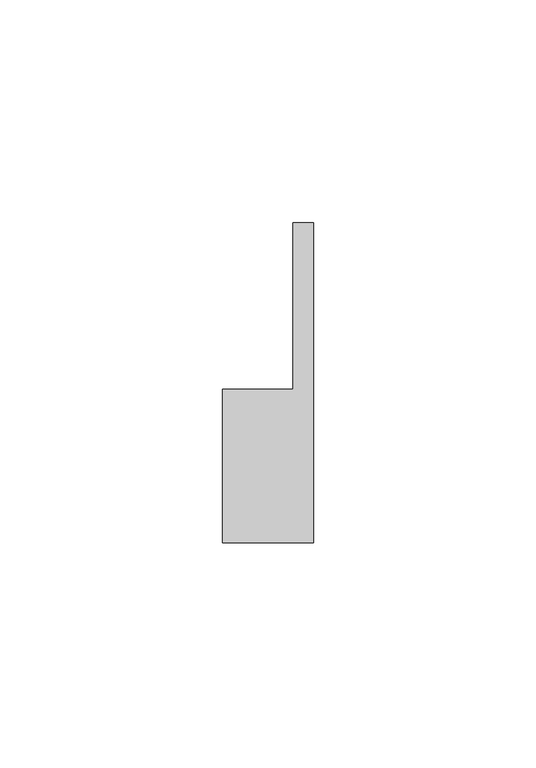
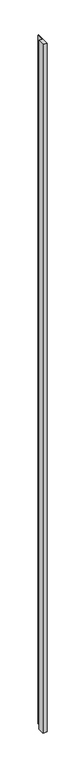
"""IFC4 building model written with IfcOpenShell, lengths in millimetres: proxy geometry, Generic Models 11:Generic Models 1:306267:Generic Models 1:306267 : Generic Models 11:Generic Models 1:306267:300405:Generic Models 1:306267:Generic Models 1:306267 : Generic Models 11:Generic Models 1:306267:300405 : Generic Models 11:Generic Models 1:306267:Generic Models 1:306267 : Generic Models 11:Generic Models 1:306267:300405:8 : Generic Models 11:Generic Models 1:306267:Generic Models 1:306267 : Generic Models 11:Generic Models 1:306267:300405:Generic Models 1:306267:Generic Models 1:306267 : Generic Models 11:Generic Models 1:306267:300405 : Generic Models 11:Generic Models 1:306267:Generic Models 1:306267 : Generic Models 11:Generic Models 1:306267:300405:300182."""

from ifc_helpers import new_model, si_unit, origin, origin_with_axes, place, context, project, spatial, polyline, outline, extrude, source, transform, mapped, element, save


def generic_models_86148c45(model_context):
    return source(origin(), model_context, "Body", "SweptSolid", [
        extrude(outline(polyline([(570447.2188081, -579043.9402915), (570447.2188081, -579006.5153982), (570451.8591519, -579006.5153982), (570451.8591519, -579078.4496134), (570431.3487584, -579078.4496134), (570431.3487584, -579043.9402915), (570447.2188081, -579043.9402915)])), origin_with_axes(), (0.0, 0.0, 1.0), 3689.35),
    ])


if __name__ == "__main__":
    model = new_model("IFC4")
    model_context = context("Model", 3, world=origin())
    ifc_project = project(units=[si_unit("LENGTHUNIT", "METRE", prefix="MILLI")], contexts=[model_context])
    site = spatial("IfcSite", under=ifc_project)
    building = spatial("IfcBuilding", under=site)
    placement = place(None, origin())
    generic_models_shape = generic_models_86148c45(model_context)
    element("IfcBuildingElementProxy", 1, Name="Generic Models 11:Generic Models 1:306267:Generic Models 1:306267 : Generic Models 11:Generic Models 1:306267:300405:Generic Models 1:306267:Generic Models 1:306267 : Generic Models 11:Generic Models 1:306267:300405 : Generic Models 11:Generic Models 1:306267:Generic Models 1:306267 : Generic Models 11:Generic Models 1:306267:300405:8 : Generic Models 11:Generic Models 1:306267:Generic Models 1:306267 : Generic Models 11:Generic Models 1:306267:300405:Generic Models 1:306267:Generic Models 1:306267 : Generic Models 11:Generic Models 1:306267:300405 : Generic Models 11:Generic Models 1:306267:Generic Models 1:306267 : Generic Models 11:Generic Models 1:306267:300405:300182", ObjectType="Generic Models 11:Generic Models 1:306267:Generic Models 1:306267 : Generic Models 11:Generic Models 1:306267:300405:Generic Models 1:306267:Generic Models 1:306267 : Generic Models 11:Generic Models 1:306267:300405 : Generic Models 11:Generic Models 1:306267:Generic Models 1:306267 : Generic Models 11:Generic Models 1:306267:300405:8 : Generic Models 11:Generic Models 1:306267:Generic Models 1:306267 : Generic Models 11:Generic Models 1:306267:300405:Generic Models 1:306267:Generic Models 1:306267 : Generic Models 11:Generic Models 1:306267:300405 : Generic Models 11:Generic Models 1:306267:Generic Models 1:306267 : Generic Models 11:Generic Models 1:306267:300405:300182", at=placement, inside=building, context=model_context, shape_type="MappedRepresentation", body=[
        mapped(generic_models_shape, transform((0.0, 0.0, 0.0), x_axis=(1.0, 0.0, 0.0), y_axis=(0.0, 1.0, 0.0), z_axis=(0.0, 0.0, 1.0))),
    ])
    save(model, "model.ifc")

# Revit data of these elements
# Type "Generic Models 11:Generic Models 1:306267:Generic Models 1:306267 : Generic Models 11:Generic Models 1:306267:300405:Generic Models 1:306267:Generic Models 1:306267 : Generic Models 11:Generic Models 1:306267:300405 : Generic Models 11:Generic Models 1:306267:Generic Models 1:306267 : Generic Models 11:Generic Models 1:306267:300405:8 : Generic Models 11:Generic Models 1:306267:Generic Models 1:306267 : Generic Models 11:Generic Models 1:306267:300405:Generic Models 1:306267:Generic Models 1:306267 : Generic Models 11:Generic Models 1:306267:300405 : Generic Models 11:Generic Models 1:306267:Generic Models 1:306267 : Generic Models 11:Generic Models 1:306267:300405:300182"
#   NameOverride = "Generic Models 11:Generic Models 1:306267:Generic Models 1:306267 : Generic Models 11:Generic Models 1:306267:300405:Generic Models 1:306267:Generic Models 1:306267 : Generic Models 11:Generic Models 1:306267:300405 : Generic Models 11:Generic Models 1:306267:Generic Models 1:306267 : Generic Models 11:Generic Models 1:306267:300405:300182"
#   ObjectTypeOverride = "Generic Models 1:306267:Generic Models 1:306267 : Generic Models 11:Generic Models 1:306267:300405 : Generic Models 11:Generic Models 1:306267:Generic Models 1:306267 : Generic Models 11:Generic Models 1:306267:300405"
#   Reference = "Generic Models 1"
#   Tag = "300182"
# Element 1 (IfcBuildingElementProxy, "Generic Models 11:Generic Models 1:306267:Generic Models 1:306267 : Generic Models 11:Generic Models 1:306267:300405:Generic Models 1:306267:Generic Models 1:306267 : Generic Models 11:Generic Models 1:306267:300405 : Generic Models 11:Generic Models 1:306267:Generic Models 1:306267 : Generic Models 11:Generic Models 1:306267:300405:8 : Generic Models 11:Generic Models 1:306267:Generic Models 1:306267 : Generic Models 11:Generic Models 1:306267:300405:Generic Models 1:306267:Generic Models 1:306267 : Generic Models 11:Generic Models 1:306267:300405 : Generic Models 11:Generic Models 1:306267:Generic Models 1:306267 : Generic Models 11:Generic Models 1:306267:300405:300182")
#   Materials on its faces: "LOW VOLUMN EXPANDABLE FOAM INSULATION"
# Materials
#   "LOW VOLUMN EXPANDABLE FOAM INSULATION": class "Unassigned", colour RGB 213 216 95, transparency 0, Cost = 0
